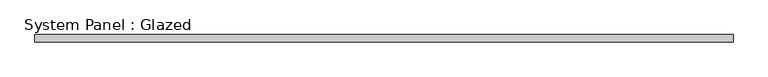
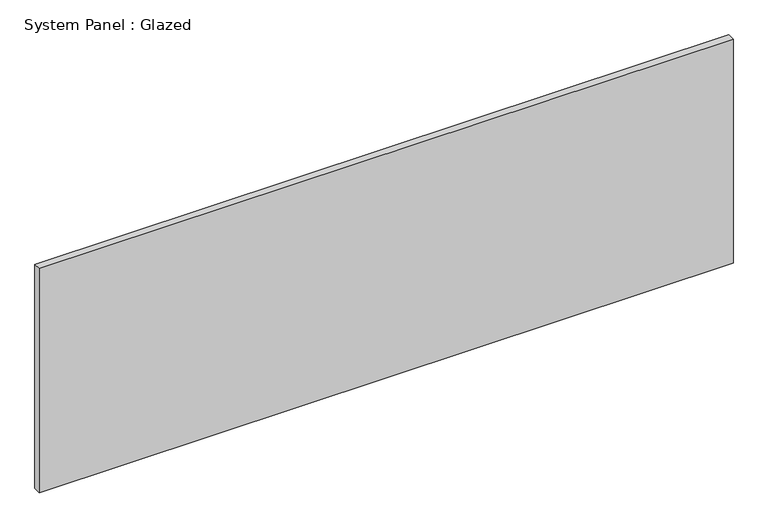
"""IFC4 building model written with IfcOpenShell, lengths in millimetres: plate geometry, System Panel : Glazed."""

from ifc_helpers import new_model, si_unit, origin, origin_with_axes, place, context, project, spatial, polyline, outline, extrude, source, transform, mapped, element, save


def system_panel_glazed_4fe69e40(model_context):
    return source(origin(), model_context, "Body", "SweptSolid", [
        extrude(outline(polyline([(1199.1815359, -44.45), (-1199.1815359, -44.45), (-1199.1815359, -19.05), (1199.1815359, -19.05), (1199.1815359, -44.45)])), origin_with_axes(), (0.0, 0.0, 1.0), 819.15),
    ])


if __name__ == "__main__":
    model = new_model("IFC4")
    model_context = context("Model", 3, world=origin())
    ifc_project = project(units=[si_unit("LENGTHUNIT", "METRE", prefix="MILLI")], contexts=[model_context])
    site = spatial("IfcSite", under=ifc_project)
    building = spatial("IfcBuilding", under=site)
    placement = place(None, origin())
    system_panel_glazed_shape = system_panel_glazed_4fe69e40(model_context)
    element("IfcPlate", 1, ObjectType="System Panel : Glazed", at=placement, inside=building, context=model_context, shape_type="MappedRepresentation", body=[
        mapped(system_panel_glazed_shape, transform((0.0, 0.0, 0.0), x_axis=(1.0, 0.0, 0.0), y_axis=(0.0, 1.0, 0.0), z_axis=(0.0, 0.0, 1.0))),
    ])
    save(model, "model.ifc")

# Revit data of these elements
# Type "System Panel : Glazed"
#   Construction Type Id = "GSP4R"
#   Analytic Construction = "1/8 in Pilkington single glazing"
#   Visual Light Transmittance = 0.9
#   Solar Heat Gain Coefficient = 0.86
#   Heat Transfer Coefficient (U) = 1.18115 BTU/(h·ft²·°F)
#   Define Thermal Properties by = 1
# Element 1 (IfcPlate, "System Panel : Glazed")
#   Materials on its faces: "Glass"
# Materials
#   "Glass": class "Glass", colour RGB 0 128 192, transparency 0.75, Description = "Soda Lime Glass", Cost = 0
